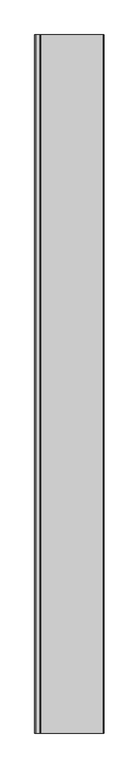
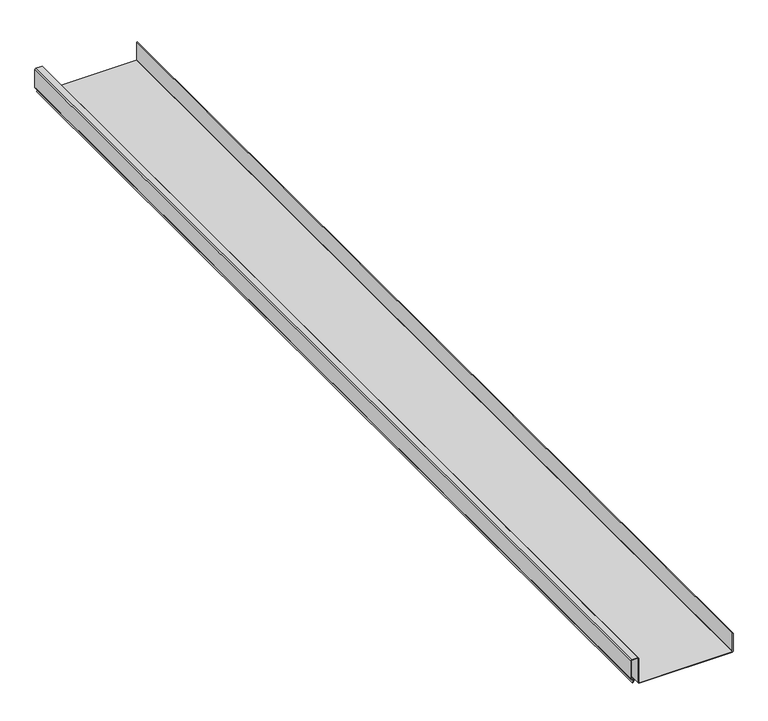
"""IFC4 building model written with IfcOpenShell, lengths in millimetres: proxy geometry, BEND PANEL001 6087 : BEND PANEL001 6087."""

from ifc_helpers import new_model, si_unit, frame, origin, place, context, project, spatial, polyline, outline, extrude, source, transform, mapped, element, save


def generic_models_8c9d74ad(model_context):
    return source(origin(), model_context, "Body", "SweptSolid", [
        extrude(outline(polyline([(42589.7865091, 5848.1043867), (42589.2833292, 5849.1834595), (42594.3520112, 5851.5470247), (42596.210073, 5850.8707455), (42598.2005361, 5846.6022357), (42599.4643694, 5845.8020635), (42634.8859537, 5845.8020635), (42636.2841216, 5847.2002314), (42636.2841216, 5857.8984229), (42634.8859537, 5859.2965908), (42585.9088212, 5859.2965908), (42584.5106533, 5860.6947587), (42584.5106533, 6041.8377287), (42585.9101309, 6043.2372063), (42623.1706509, 6043.2372063), (42623.1706509, 6042.0465813), (42586.4033039, 6042.0465813), (42585.7012783, 6041.3445557), (42585.7012783, 5861.1879317), (42586.4019942, 5860.4872158), (42635.3791267, 5860.4872158), (42637.4747466, 5858.3915959), (42637.4747466, 5846.7070584), (42635.3791267, 5844.6114385), (42599.1191461, 5844.6114385), (42597.268896, 5845.7828894), (42595.3394273, 5849.920598), (42594.4082245, 5850.259528), (42589.7865091, 5848.1043867)])), frame((0.0, -1052.8906574, 0.0), z_axis=(0.0, 1.0, 0.0), x_axis=(0.0, 0.0, 1.0)), (0.0, 0.0, 1.0), 1999.85),
    ])


if __name__ == "__main__":
    model = new_model("IFC4")
    model_context = context("Model", 3, world=origin())
    ifc_project = project(units=[si_unit("LENGTHUNIT", "METRE", prefix="MILLI")], contexts=[model_context])
    site = spatial("IfcSite", under=ifc_project)
    building = spatial("IfcBuilding", under=site)
    placement = place(None, origin())
    generic_models_shape = generic_models_8c9d74ad(model_context)
    element("IfcBuildingElementProxy", 1, Name="BEND PANEL001 6087 : BEND PANEL001 6087", ObjectType="BEND PANEL001 6087 : BEND PANEL001 6087", at=placement, inside=building, context=model_context, shape_type="MappedRepresentation", body=[
        mapped(generic_models_shape, transform((0.0, 0.0, 0.0), x_axis=(1.0, 0.0, 0.0), y_axis=(0.0, 1.0, 0.0), z_axis=(0.0, 0.0, 1.0))),
    ])
    save(model, "model.ifc")

# Revit data of these elements
# Type "BEND PANEL001 6087 : BEND PANEL001 6087"
#   NameOverride = "BEND PANEL001"
# Element 1 (IfcBuildingElementProxy, "BEND PANEL001 6087 : BEND PANEL001 6087")
#   Materials on its faces: "STANDING SEAM METAL ROOF FOLLOW MANU. RECOMMENDED EDGE/TRANSITION DETAILS"
# Materials
#   "STANDING SEAM METAL ROOF FOLLOW MANU. RECOMMENDED EDGE/TRANSITION DETAILS": class "Unassigned", colour RGB 128 128 128, transparency 0
